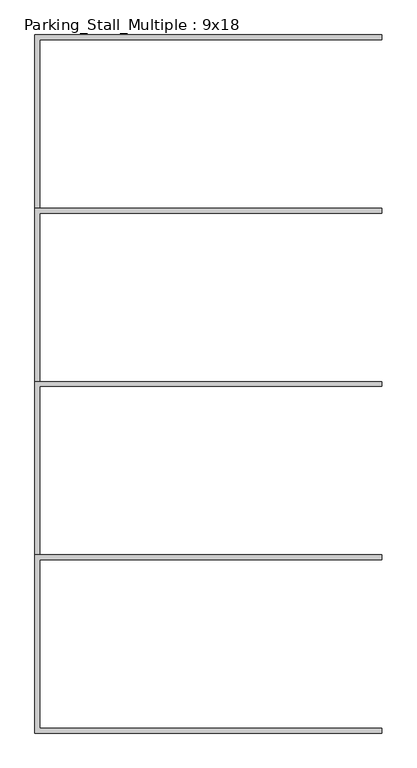
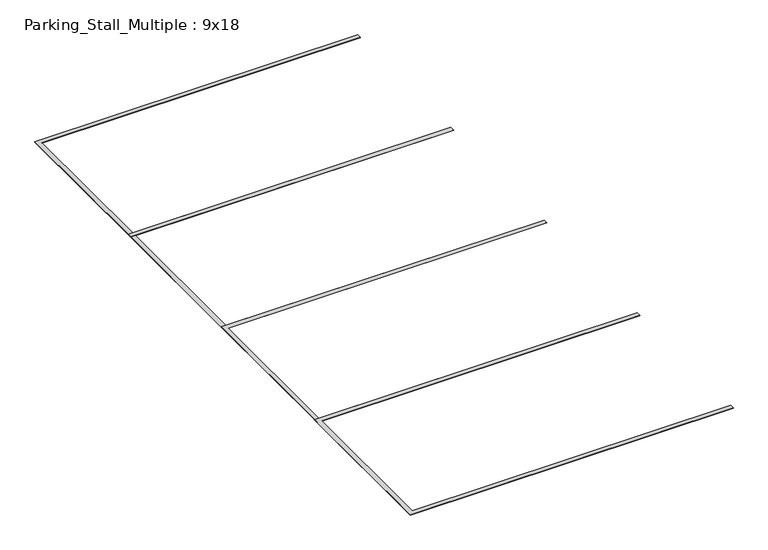
"""IFC4 building model written with IfcOpenShell, lengths in millimetres: proxy geometry, Parking_Stall_Multiple : 9x18."""

import ifcopenshell
import ifcopenshell.guid

model = None  # the IFC model being written
_history = None  # IfcOwnerHistory: only IFC2X3 demands one
_inside = {}  # id of a spatial element -> (the spatial element, [elements in it])
_under = {}  # id of a project, library or spatial element -> (it, [spatial elements below it])
_declared = {}  # id of a project -> (the project, [libraries it declares])
_typed = {}  # id of a type object -> (the type object, [elements of that type])
_made_of = {}  # id of a material, layer set ... -> (it, [elements and type objects made of it])


def new_model(schema):
    """Start an empty IFC model of exactly this schema.

    Asked for "IFC4X3", IfcOpenShell would pick the latest addendum, in which some entities
    have other attributes; the version numbers below select the first issue.
    IFC2X3 requires an IfcOwnerHistory on every rooted entity: one is made here for all.
    """
    global model, _history
    if schema == "IFC4X3":
        model = ifcopenshell.file(schema_version=(4, 3, 0, 0))
    else:
        model = ifcopenshell.file(schema=schema)
    _inside.clear()
    _under.clear()
    _declared.clear()
    _typed.clear()
    _made_of.clear()
    _history = None
    if model.schema == "IFC2X3":
        org = make("IfcOrganization", Name="unknown")
        user = make(
            "IfcPersonAndOrganization",
            ThePerson=make("IfcPerson", FamilyName="unknown"),
            TheOrganization=org,
        )
        app = make(
            "IfcApplication",
            ApplicationDeveloper=org,
            Version="unknown",
            ApplicationFullName="unknown",
            ApplicationIdentifier="unknown",
        )
        _history = make(
            "IfcOwnerHistory",
            OwningUser=user,
            OwningApplication=app,
            ChangeAction="ADDED",
            CreationDate=0,
        )
    return model


def make(cls, **values):
    """One entity of the class cls with the attributes given. An attribute that is None is left unset."""
    return model.create_entity(
        cls, **{name: value for name, value in values.items() if value is not None}
    )


def rooted(cls, **values):
    """An entity with a GlobalId (a new one), such as an element, a storey or a relation."""
    return make(cls, GlobalId=ifcopenshell.guid.new(), OwnerHistory=_history, **values)


def si_unit(unit_type, name, prefix=None):
    """IfcSIUnit, for example si_unit("LENGTHUNIT", "METRE", prefix="MILLI")."""
    return make("IfcSIUnit", UnitType=unit_type, Prefix=prefix, Name=name)


def assignment(units):
    """IfcUnitAssignment: the units of a project."""
    return None if units is None else make("IfcUnitAssignment", Units=units)


def point(xyz):
    """IfcCartesianPoint."""
    return None if xyz is None else make("IfcCartesianPoint", Coordinates=xyz)


def direction(xyz):
    """IfcDirection."""
    return None if xyz is None else make("IfcDirection", DirectionRatios=xyz)


def frame(location, z_axis=None, x_axis=None):
    """IfcAxis2Placement3D, a coordinate frame: its origin and axes. An axis left out is left unset."""
    return make(
        "IfcAxis2Placement3D",
        Location=point(location),
        Axis=direction(z_axis),
        RefDirection=direction(x_axis),
    )


def origin():
    """The frame at (0, 0, 0) with its axes left unset."""
    return frame((0.0, 0.0, 0.0))


def origin_with_axes():
    """The frame at (0, 0, 0) with the z axis (0, 0, 1) and the x axis (1, 0, 0) written out."""
    return frame((0.0, 0.0, 0.0), z_axis=(0.0, 0.0, 1.0), x_axis=(1.0, 0.0, 0.0))


def place(relative_to, where):
    """IfcLocalPlacement: puts the frame where relative to a parent placement (None: the world)."""
    return make(
        "IfcLocalPlacement", PlacementRelTo=relative_to, RelativePlacement=where
    )


def context(
    kind, dimensions, precision=None, world=None, true_north=None, identifier=None
):
    """IfcGeometricRepresentationContext, for example the 3D "Model" context."""
    return make(
        "IfcGeometricRepresentationContext",
        ContextIdentifier=identifier,
        ContextType=kind,
        CoordinateSpaceDimension=dimensions,
        Precision=precision,
        WorldCoordinateSystem=world,
        TrueNorth=true_north,
    )


def project(units=None, contexts=None):
    """IfcProject with its units and contexts."""
    return rooted(
        "IfcProject",
        Name="project",
        RepresentationContexts=contexts,
        UnitsInContext=assignment(units),
    )


def spatial(cls, under=None, at=None, **own):
    """A site, building, storey or space (cls), placed at a placement, below another one or the project."""
    s = rooted(cls, ObjectPlacement=at, **own)
    if under is not None:
        _under.setdefault(under.id(), (under, []))[1].append(s)
    return s


def polyline(points):
    """IfcPolyline through the points."""
    return make("IfcPolyline", Points=[point(p) for p in points])


def outline(outer, holes=None, kind="AREA"):
    """IfcArbitraryClosedProfileDef: a profile drawn as a closed curve; with holes, ...WithVoids."""
    if holes is None:
        return make("IfcArbitraryClosedProfileDef", ProfileType=kind, OuterCurve=outer)
    return make(
        "IfcArbitraryProfileDefWithVoids",
        ProfileType=kind,
        OuterCurve=outer,
        InnerCurves=holes,
    )


def extrude(swept, where, along, depth):
    """IfcExtrudedAreaSolid: the profile swept, set in the frame where, extruded along a direction by depth."""
    return make(
        "IfcExtrudedAreaSolid",
        SweptArea=swept,
        Position=where,
        ExtrudedDirection=direction(along),
        Depth=depth,
    )


def shape(context_of_items, identifier, shape_type, items):
    """IfcShapeRepresentation: the items that make up one representation, for example the "Body"."""
    return make(
        "IfcShapeRepresentation",
        ContextOfItems=context_of_items,
        RepresentationIdentifier=identifier,
        RepresentationType=shape_type,
        Items=items,
    )


def source(mapping_origin, context_of_items, identifier, shape_type, items):
    """IfcRepresentationMap: a shape defined once, which mapped items show again and again."""
    return make(
        "IfcRepresentationMap",
        MappingOrigin=mapping_origin,
        MappedRepresentation=shape(context_of_items, identifier, shape_type, items),
    )


def transform(
    local_origin,
    x_axis=None,
    y_axis=None,
    z_axis=None,
    scale=None,
    scale2=None,
    scale3=None,
    uniform=True,
):
    """IfcCartesianTransformationOperator3D, or its non-uniform kind. x_axis, y_axis, z_axis: its Axis1, 2, 3."""
    if uniform:
        return make(
            "IfcCartesianTransformationOperator3D",
            Axis1=direction(x_axis),
            Axis2=direction(y_axis),
            LocalOrigin=point(local_origin),
            Scale=scale,
            Axis3=direction(z_axis),
        )
    return make(
        "IfcCartesianTransformationOperator3DnonUniform",
        Axis1=direction(x_axis),
        Axis2=direction(y_axis),
        LocalOrigin=point(local_origin),
        Scale=scale,
        Axis3=direction(z_axis),
        Scale2=scale2,
        Scale3=scale3,
    )


def mapped(mapping_source, mapping_target):
    """IfcMappedItem: shows the shape of a source again, moved by a transform."""
    return make(
        "IfcMappedItem", MappingSource=mapping_source, MappingTarget=mapping_target
    )


def made_of(thing, what):
    """Note that an element or type object is made of a material, layer set ...; save() writes the relation."""
    if what is not None:
        _made_of.setdefault(what.id(), (what, []))[1].append(thing)
    return thing


def element(
    cls,
    number,
    at=None,
    inside=None,
    cuts=None,
    type_object=None,
    material=None,
    context=None,
    identifier="Body",
    shape_type=None,
    held_by="IfcProductDefinitionShape",
    body=None,
    shapes=None,
    **own,
):
    """One element of the class cls, such as IfcWall. Its Tag is "e" and its number.

    at: its placement. inside: the storey or other place that contains it. cuts: it is an
    opening in that element (IfcRelVoidsElement). A single representation is given by context,
    identifier, shape_type and body (its items); several are given by shapes. held_by: the class
    of the entity that holds the representations. save() writes the other relations.
    """
    e = rooted(cls, Tag="e%d" % number, ObjectPlacement=at, **own)
    if body is not None:
        shapes = [shape(context, identifier, shape_type, body)]
    if shapes is not None:
        e.Representation = make(held_by, Representations=shapes)
    if inside is not None:
        _inside.setdefault(inside.id(), (inside, []))[1].append(e)
    if cuts is not None:
        rooted(
            "IfcRelVoidsElement", RelatingBuildingElement=cuts, RelatedOpeningElement=e
        )
    if type_object is not None:
        _typed.setdefault(type_object.id(), (type_object, []))[1].append(e)
    return made_of(e, material)


def aggregate(whole, parts):
    """IfcRelAggregates: a whole, such as a stair, and the parts it consists of."""
    return rooted("IfcRelAggregates", RelatingObject=whole, RelatedObjects=parts)


def save(model, path):
    """Write the relations noted so far, then the file.

    IfcRelAggregates (storeys below a building ...), IfcRelContainedInSpatialStructure (elements
    in a storey), IfcRelDefinesByType, IfcRelAssociatesMaterial and IfcRelDeclares: one each for
    every whole, place, type object, material and project.
    """
    for whole, parts in _under.values():
        aggregate(whole, parts)
    for where, things in _inside.values():
        rooted(
            "IfcRelContainedInSpatialStructure",
            RelatedElements=things,
            RelatingStructure=where,
        )
    for kind, things in _typed.values():
        rooted("IfcRelDefinesByType", RelatedObjects=things, RelatingType=kind)
    for what, things in _made_of.values():
        rooted("IfcRelAssociatesMaterial", RelatedObjects=things, RelatingMaterial=what)
    for by, libraries in _declared.values():
        rooted("IfcRelDeclares", RelatingContext=by, RelatedDefinitions=libraries)
    model.write(path)


def parking_stall_multiple_9x18_c96fd294(model_context):
    return source(origin(), model_context, "Body", "SweptSolid", [
        extrude(outline(polyline([(5486.4, -8229.6), (5486.4, -8305.8), (76.2, -8305.8), (76.2, -10972.8), (5486.4, -10972.8), (5486.4, -11049.0), (0.0, -11049.0), (0.0, -8229.6), (5486.4, -8229.6)])), origin_with_axes(), (0.0, 0.0, 1.0), 6.35),
        extrude(outline(polyline([(5486.4, -5486.4), (5486.4, -5562.6), (76.2, -5562.6), (76.2, -8229.6), (5486.4, -8229.6), (5486.4, -8305.8), (0.0, -8305.8), (0.0, -5486.4), (5486.4, -5486.4)])), origin_with_axes(), (0.0, 0.0, 1.0), 6.35),
        extrude(outline(polyline([(5486.4, -2743.2), (5486.4, -2819.4), (76.2, -2819.4), (76.2, -5486.4), (5486.4, -5486.4), (5486.4, -5562.6), (0.0, -5562.6), (0.0, -2743.2), (5486.4, -2743.2)])), origin_with_axes(), (0.0, 0.0, 1.0), 6.35),
        extrude(outline(polyline([(5486.4, 0.0), (5486.4, -76.2), (76.2, -76.2), (76.2, -2743.2), (5486.4, -2743.2), (5486.4, -2819.4), (0.0, -2819.4), (0.0, 0.0), (5486.4, 0.0)])), origin_with_axes(), (0.0, 0.0, 1.0), 6.35),
    ])


if __name__ == "__main__":
    model = new_model("IFC4")
    model_context = context("Model", 3, world=origin())
    ifc_project = project(units=[si_unit("LENGTHUNIT", "METRE", prefix="MILLI")], contexts=[model_context])
    site = spatial("IfcSite", under=ifc_project)
    building = spatial("IfcBuilding", under=site)
    placement = place(None, origin())
    parking_stall_multiple_9x18_shape = parking_stall_multiple_9x18_c96fd294(model_context)
    element("IfcBuildingElementProxy", 1, Name="Parking_Stall_Multiple : 9x18", ObjectType="Parking_Stall_Multiple : 9x18", at=placement, inside=building, context=model_context, shape_type="MappedRepresentation", body=[
        mapped(parking_stall_multiple_9x18_shape, transform((0.0, 0.0, 0.0), x_axis=(1.0, 0.0, 0.0), y_axis=(0.0, 1.0, 0.0), z_axis=(0.0, 0.0, 1.0))),
    ])
    save(model, "model.ifc")

# Revit data of these elements
# Type "Parking_Stall_Multiple : 9x18"
#   Parking_Width_M = 9' - 0"
#   Parking_Run_Length [instance default] = 65' - 0"
#   Parking_Line_Width = 0' - 3"
#   Parking_Length_M = 18' - 0"
#   Single_Parking_Visibility [instance default] = no
#   Parking_ADA_Symbol = no
#   ParkingUnitsArray [instance default] = 7
#   ParkingUnits [instance default] = 7
#   Multiple_Parking_Visibility [instance default] = yes
#   Parking_Line_Material = none
# Element 1 (IfcBuildingElementProxy, "Parking_Stall_Multiple : 9x18")
#   Parking_Run_Length = 36' - 0.74097"
#   ParkingUnitsArray = 4
#   ParkingUnits = 4
